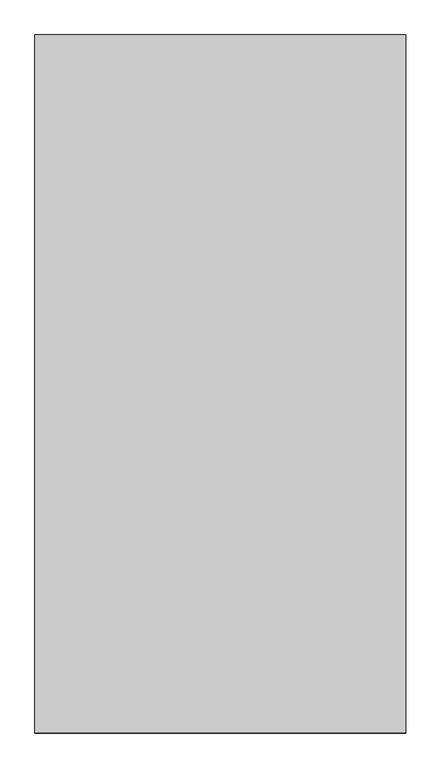
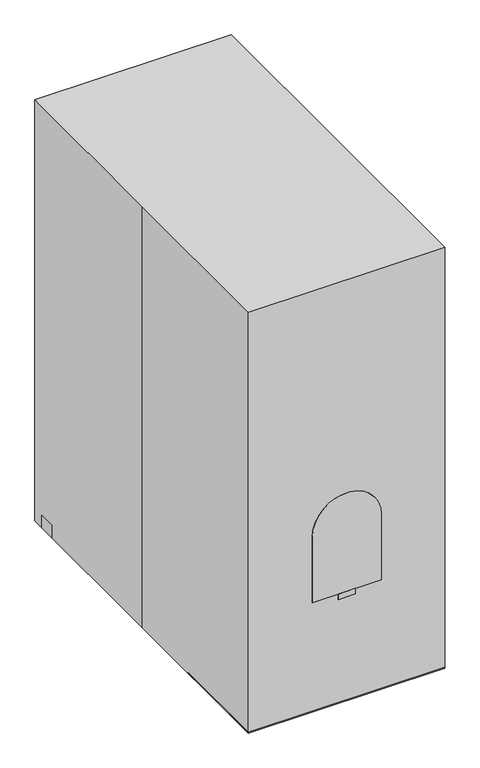
"""IFC4 building model written with IfcOpenShell, lengths in millimetres: proxy geometry, M8133 - Ergometer, Upper Body : M8133 - Ergometer, Upper Body."""

from ifc_helpers import new_model, si_unit, point, frame, frame_2d, origin, origin_with_axes, place, context, project, spatial, polyline, circle_curve, trimmed, segment, composite_curve, outline, extrude, faceted_brep, source, transform, mapped, element, save
from ifc_brep_helpers import plane_surface, cylinder_surface, revolved_surface, advanced_brep


def specialty_equipment_9e477837(model_context):
    return source(origin(), model_context, "Body", "SolidModel", [
        faceted_brep([(-152.4, -762.0, 457.2), (152.4, -762.0, 457.2), (152.4, -762.0, 508.0), (38.1, -762.0, 508.0), (38.1, -762.0, 482.6226424), (-38.1, -762.0, 482.6226424), (-38.1, -762.0, 508.0), (-152.4, -762.0, 508.0), (-152.4, -457.2, 457.2), (-152.4, -457.2, 508.0), (152.4, -457.2, 508.0), (152.4, -457.2, 457.2), (-38.1, -812.8, 508.0), (38.1, -812.8, 508.0), (-38.1, -812.8, 482.6226424), (38.1, -812.8, 482.6226424)], [[[0, 1, 2, 3, 4, 5, 6, 7]], [[8, 9, 10, 11]], [[1, 0, 8, 11]], [[2, 1, 11, 10]], [[10, 9, 7, 6, 12, 13, 3, 2]], [[0, 7, 9, 8]], [[14, 5, 4, 15]], [[13, 12, 14, 15]], [[3, 13, 15, 4]], [[12, 6, 5, 14]]]),
        advanced_brep(
        [(-76.2, 42.1480335, 1174.2765056), (-76.2, 59.4642449, 1191.592717), (-76.2, 212.6832937, 1038.3736683), (-76.2, 195.3670823, 1021.0574568), (-76.2, 46.8398769, 1180.5508736), (-76.2, 59.5398769, 1180.5508736), (-76.2, 207.9914503, 1032.0993003), (-76.2, 195.2914503, 1032.0993003), (-63.5, 42.1480335, 1174.2765056), (-63.5, 195.3670823, 1021.0574568), (-63.5, 212.6832937, 1038.3736683), (-63.5, 59.4642449, 1191.592717), (-63.5, 46.8398769, 1180.5508736), (-63.5, 59.5398769, 1180.5508736), (-165.1, 207.9914503, 1032.0993003), (-165.1, 195.2914503, 1032.0993003)],
        [
            (0, 1, circle_curve(frame((-76.2, 53.1898769, 1180.5508736), z_axis=(-1.0, 0.0, 0.0), x_axis=(0.0, 1.0, 0.0)), 12.7)),
            (1, 2),
            (2, 3, circle_curve(frame((-76.2, 201.6414503, 1032.0993003), z_axis=(-1.0, 0.0, 0.0), x_axis=(0.0, 1.0, 0.0)), 12.7)),
            (3, 0),
            (4, 5, circle_curve(frame((-76.2, 53.1898769, 1180.5508736), z_axis=(1.0, 0.0, 0.0), x_axis=(0.0, 1.0, 0.0)), 6.35)),
            (5, 4, circle_curve(frame((-76.2, 53.1898769, 1180.5508736), z_axis=(1.0, 0.0, 0.0), x_axis=(0.0, 1.0, 0.0)), 6.35)),
            (6, 7, circle_curve(frame((-76.2, 201.6414503, 1032.0993003), z_axis=(1.0, 0.0, 0.0), x_axis=(0.0, 1.0, 0.0)), 6.35)),
            (7, 6, circle_curve(frame((-76.2, 201.6414503, 1032.0993003), z_axis=(1.0, 0.0, 0.0), x_axis=(0.0, 1.0, 0.0)), 6.35)),
            (8, 9),
            (9, 10, circle_curve(frame((-63.5, 201.6414503, 1032.0993003), z_axis=(1.0, 0.0, 0.0), x_axis=(0.0, 1.0, 0.0)), 12.7)),
            (10, 11),
            (11, 8, circle_curve(frame((-63.5, 53.1898769, 1180.5508736), z_axis=(1.0, 0.0, 0.0), x_axis=(0.0, 1.0, 0.0)), 12.7)),
            (12, 13, circle_curve(frame((-63.5, 53.1898769, 1180.5508736), z_axis=(-1.0, 0.0, 0.0), x_axis=(0.0, 1.0, 0.0)), 6.35)),
            (13, 12, circle_curve(frame((-63.5, 53.1898769, 1180.5508736), z_axis=(-1.0, 0.0, 0.0), x_axis=(0.0, 1.0, 0.0)), 6.35)),
            (3, 9),
            (8, 0),
            (2, 10),
            (1, 11),
            (5, 13),
            (12, 4),
            (14, 15, circle_curve(frame((-165.1, 201.6414503, 1032.0993003), z_axis=(-1.0, 0.0, 0.0), x_axis=(0.0, 1.0, 0.0)), 6.35)),
            (15, 14, circle_curve(frame((-165.1, 201.6414503, 1032.0993003), z_axis=(-1.0, 0.0, 0.0), x_axis=(0.0, 1.0, 0.0)), 6.35)),
            (15, 7),
            (6, 14),
        ],
        [
            plane_surface(frame((-76.2, 65.8898769, 1180.5508736), z_axis=(-1.0, 0.0, 0.0), x_axis=(0.0, 0.0, -1.0))),
            plane_surface(frame((-63.5, 65.8898769, 1180.5508736), z_axis=(1.0, 0.0, 0.0), x_axis=(0.0, 0.0, 1.0))),
            plane_surface(frame((-76.2, 195.3670823, 1021.0574568), z_axis=(0.0, -0.7071067811865492, -0.7071067811865458), x_axis=(1.0, 0.0, 0.0))),
            cylinder_surface(frame((-63.5, 201.6414503, 1032.0993003), z_axis=(-1.0, 0.0, 0.0), x_axis=(0.0, 1.0, 0.0)), 12.7),
            plane_surface(frame((-76.2, 59.4642449, 1191.592717), z_axis=(0.0, 0.7071067811865492, 0.7071067811865458), x_axis=(1.0, 0.0, 0.0))),
            cylinder_surface(frame((-63.5, 53.1898769, 1180.5508736), z_axis=(-1.0, 0.0, 0.0), x_axis=(0.0, 1.0, 0.0)), 12.7),
            revolved_surface(polyline([(-63.5, 59.5398769, 1180.5508736), (-76.2, 59.5398769, 1180.5508736)]), (0.0, 53.1898769, 1180.5508736), (1.0, 0.0, 0.0)),
            plane_surface(frame((-165.1, 207.9914503, 1032.0993003), z_axis=(-1.0, 0.0, 0.0), x_axis=(0.0, 0.0, -1.0))),
            cylinder_surface(frame((-63.5, 201.6414503, 1032.0993003), z_axis=(-1.0, 0.0, 0.0), x_axis=(0.0, 1.0, 0.0)), 6.35),
        ],
        [
            (0, [[1, 2, 3, 4], [5, 6], [7, 8]]),
            (1, [[9, 10, 11, 12], [13, 14]]),
            (2, [[-4, 15, -9, 16]]),
            (3, [[-3, 17, -10, -15]]),
            (4, [[-2, 18, -11, -17]]),
            (5, [[-1, -16, -12, -18]]),
            (6, [[-6, 19, -13, 20]]),
            (6, [[-5, -20, -14, -19]]),
            (7, [[21, 22]]),
            (8, [[-22, 23, -7, 24]]),
            (8, [[-21, -24, -8, -23]]),
        ],
    ),
        advanced_brep(
        [(165.1, 207.9914503, 1032.0993003), (165.1, 195.2914503, 1032.0993003), (63.5, 42.1480335, 1174.2765056), (63.5, 59.4642449, 1191.592717), (63.5, 212.6832937, 1038.3736683), (63.5, 195.3670823, 1021.0574568), (63.5, 46.8398769, 1180.5508736), (63.5, 59.5398769, 1180.5508736), (76.2, 207.9914503, 1032.0993003), (76.2, 195.2914503, 1032.0993003), (76.2, 42.1480335, 1174.2765056), (76.2, 195.3670823, 1021.0574568), (76.2, 212.6832937, 1038.3736683), (76.2, 59.4642449, 1191.592717), (76.2, 46.8398769, 1180.5508736), (76.2, 59.5398769, 1180.5508736)],
        [
            (0, 1, circle_curve(frame((165.1, 201.6414503, 1032.0993003), z_axis=(1.0, 0.0, 0.0), x_axis=(0.0, 1.0, 0.0)), 6.35)),
            (1, 0, circle_curve(frame((165.1, 201.6414503, 1032.0993003), z_axis=(1.0, 0.0, 0.0), x_axis=(0.0, 1.0, 0.0)), 6.35)),
            (2, 3, circle_curve(frame((63.5, 53.1898769, 1180.5508736), z_axis=(-1.0, 0.0, 0.0), x_axis=(0.0, 1.0, 0.0)), 12.7)),
            (3, 4),
            (4, 5, circle_curve(frame((63.5, 201.6414503, 1032.0993003), z_axis=(-1.0, 0.0, 0.0), x_axis=(0.0, 1.0, 0.0)), 12.7)),
            (5, 2),
            (6, 7, circle_curve(frame((63.5, 53.1898769, 1180.5508736), z_axis=(1.0, 0.0, 0.0), x_axis=(0.0, 1.0, 0.0)), 6.35)),
            (7, 6, circle_curve(frame((63.5, 53.1898769, 1180.5508736), z_axis=(1.0, 0.0, 0.0), x_axis=(0.0, 1.0, 0.0)), 6.35)),
            (0, 8),
            (8, 9, circle_curve(frame((76.2, 201.6414503, 1032.0993003), z_axis=(1.0, 0.0, 0.0), x_axis=(0.0, 1.0, 0.0)), 6.35)),
            (9, 1),
            (9, 8, circle_curve(frame((76.2, 201.6414503, 1032.0993003), z_axis=(1.0, 0.0, 0.0), x_axis=(0.0, 1.0, 0.0)), 6.35)),
            (10, 11),
            (11, 12, circle_curve(frame((76.2, 201.6414503, 1032.0993003), z_axis=(1.0, 0.0, 0.0), x_axis=(0.0, 1.0, 0.0)), 12.7)),
            (12, 13),
            (13, 10, circle_curve(frame((76.2, 53.1898769, 1180.5508736), z_axis=(1.0, 0.0, 0.0), x_axis=(0.0, 1.0, 0.0)), 12.7)),
            (14, 15, circle_curve(frame((76.2, 53.1898769, 1180.5508736), z_axis=(-1.0, 0.0, 0.0), x_axis=(0.0, 1.0, 0.0)), 6.35)),
            (15, 14, circle_curve(frame((76.2, 53.1898769, 1180.5508736), z_axis=(-1.0, 0.0, 0.0), x_axis=(0.0, 1.0, 0.0)), 6.35)),
            (10, 2),
            (5, 11),
            (4, 12),
            (3, 13),
            (14, 6),
            (7, 15),
        ],
        [
            plane_surface(frame((165.1, 207.9914503, 1032.0993003), z_axis=(1.0, 0.0, 0.0), x_axis=(0.0, 0.0, 1.0))),
            plane_surface(frame((63.5, 207.9914503, 1032.0993003), z_axis=(-1.0, 0.0, 0.0), x_axis=(0.0, 0.0, -1.0))),
            cylinder_surface(frame((63.5, 201.6414503, 1032.0993003), z_axis=(1.0, 0.0, 0.0), x_axis=(0.0, 1.0, 0.0)), 6.35),
            plane_surface(frame((76.2, 51.6829843, 1164.7415548), z_axis=(1.0, 0.0, 0.0), x_axis=(0.0, 0.7071067811865458, -0.7071067811865492))),
            plane_surface(frame((76.2, 42.1480335, 1174.2765056), z_axis=(0.0, -0.7071067811865492, -0.7071067811865458), x_axis=(-1.0, 0.0, 0.0))),
            cylinder_surface(frame((63.5, 201.6414503, 1032.0993003), z_axis=(1.0, 0.0, 0.0), x_axis=(0.0, 1.0, 0.0)), 12.7),
            plane_surface(frame((76.2, 212.6832937, 1038.3736683), z_axis=(0.0, 0.7071067811865492, 0.7071067811865458), x_axis=(-1.0, 0.0, 0.0))),
            cylinder_surface(frame((63.5, 53.1898769, 1180.5508736), z_axis=(1.0, 0.0, 0.0), x_axis=(0.0, 1.0, 0.0)), 12.7),
            revolved_surface(polyline([(63.5, 59.5398769, 1180.5508736), (76.2, 59.5398769, 1180.5508736)]), (0.0, 53.1898769, 1180.5508736), (-1.0, 0.0, 0.0)),
        ],
        [
            (0, [[1, 2]]),
            (1, [[3, 4, 5, 6], [7, 8]]),
            (2, [[-1, 9, 10, 11]]),
            (2, [[-2, -11, 12, -9]]),
            (3, [[13, 14, 15, 16], [-10, -12], [17, 18]]),
            (4, [[-13, 19, -6, 20]]),
            (5, [[-14, -20, -5, 21]]),
            (6, [[-15, -21, -4, 22]]),
            (7, [[-16, -22, -3, -19]]),
            (8, [[-17, 23, -8, 24]]),
            (8, [[-18, -24, -7, -23]]),
        ],
    ),
        advanced_brep(
        [(50.8, 0.0, 1270.0), (50.8, 0.0, 1066.8), (50.8, 475.1958334, 1117.6), (50.8, 406.4, 1270.0), (50.8, 487.68, 1432.56), (50.8, 468.63, 1426.21), (50.8, 196.9503327, 1426.21), (50.8, 171.5503327, 1400.81), (50.8, 171.5503327, 1327.1834442), (50.8, 59.5398769, 1180.5508736), (50.8, 46.8398769, 1180.5508736), (-50.8, 475.1958334, 1117.6), (-50.8, 0.0, 1066.8), (-50.8, 0.0, 1270.0), (-50.8, 171.5503327, 1327.1834442), (-50.8, 171.5503327, 1400.81), (-50.8, 196.9503327, 1426.21), (-50.8, 468.63, 1426.21), (-50.8, 487.68, 1432.56), (-50.8, 406.4, 1270.0), (-50.8, 46.8398769, 1180.5508736), (-50.8, 59.5398769, 1180.5508736), (76.2, 406.4, 1270.0), (76.2, 812.8, 1270.0), (-76.2, 406.4, 1270.0), (-76.2, 812.8, 1270.0), (63.5, 486.8027128, 1108.1016793), (63.5, 541.769184, 1078.455696), (-63.5, 541.769184, 1078.455696), (-63.5, 486.8027128, 1108.1016793), (63.5, 634.9505562, 53.975), (63.5, 685.7505562, 53.975), (-63.5, 685.7505562, 53.975), (-63.5, 634.9505562, 53.975), (76.2, 46.8398769, 1180.5508736), (76.2, 59.5398769, 1180.5508736), (-76.2, 46.8398769, 1180.5508736), (-76.2, 59.5398769, 1180.5508736)],
        [
            (0, 1, circle_curve(frame((50.8, 33.8666667, 1168.4), z_axis=(1.0, 0.0, 0.0), x_axis=(0.0, 1.0, 0.0)), 107.0958034)),
            (1, 2),
            (2, 3, circle_curve(frame((50.8, 609.6, 1270.0), z_axis=(-1.0, 0.0, 0.0), x_axis=(0.0, 1.0, 0.0)), 203.2)),
            (3, 4, circle_curve(frame((50.8, 609.6, 1270.0), z_axis=(-1.0, 0.0, 0.0), x_axis=(0.0, 1.0, 0.0)), 203.2)),
            (4, 5),
            (5, 6),
            (6, 7, circle_curve(frame((50.8, 196.9503327, 1400.81), z_axis=(1.0, 0.0, 0.0), x_axis=(0.0, 1.0, 0.0)), 25.4)),
            (7, 8),
            (8, 0),
            (9, 10, circle_curve(frame((50.8, 53.1898769, 1180.5508736), z_axis=(-1.0, 0.0, 0.0), x_axis=(0.0, 1.0, 0.0)), 6.35)),
            (10, 9, circle_curve(frame((50.8, 53.1898769, 1180.5508736), z_axis=(-1.0, 0.0, 0.0), x_axis=(0.0, 1.0, 0.0)), 6.35)),
            (11, 12),
            (12, 13, circle_curve(frame((-50.8, 33.8666667, 1168.4), z_axis=(-1.0, 0.0, 0.0), x_axis=(0.0, 1.0, 0.0)), 107.0958034)),
            (13, 14),
            (14, 15),
            (15, 16, circle_curve(frame((-50.8, 196.9503327, 1400.81), z_axis=(-1.0, 0.0, 0.0), x_axis=(0.0, 1.0, 0.0)), 25.4)),
            (16, 17),
            (17, 18),
            (18, 19, circle_curve(frame((-50.8, 609.6, 1270.0), z_axis=(1.0, 0.0, 0.0), x_axis=(0.0, 1.0, 0.0)), 203.2)),
            (19, 11, circle_curve(frame((-50.8, 609.6, 1270.0), z_axis=(1.0, 0.0, 0.0), x_axis=(0.0, 1.0, 0.0)), 203.2)),
            (20, 21, circle_curve(frame((-50.8, 53.1898769, 1180.5508736), z_axis=(1.0, 0.0, 0.0), x_axis=(0.0, 1.0, 0.0)), 6.35)),
            (21, 20, circle_curve(frame((-50.8, 53.1898769, 1180.5508736), z_axis=(1.0, 0.0, 0.0), x_axis=(0.0, 1.0, 0.0)), 6.35)),
            (13, 0),
            (8, 14),
            (4, 18),
            (17, 5),
            (12, 1),
            (11, 2),
            (22, 23, circle_curve(frame((76.2, 609.6, 1270.0), z_axis=(1.0, 0.0, 0.0), x_axis=(0.0, 1.0, 0.0)), 203.2)),
            (23, 22, circle_curve(frame((76.2, 609.6, 1270.0), z_axis=(1.0, 0.0, 0.0), x_axis=(0.0, 1.0, 0.0)), 203.2)),
            (24, 25, circle_curve(frame((-76.2, 609.6, 1270.0), z_axis=(-1.0, 0.0, 0.0), x_axis=(0.0, 1.0, 0.0)), 203.2)),
            (25, 24, circle_curve(frame((-76.2, 609.6, 1270.0), z_axis=(-1.0, 0.0, 0.0), x_axis=(0.0, 1.0, 0.0)), 203.2)),
            (22, 3),
            (19, 24),
            (25, 23),
            (26, 27, circle_curve(frame((63.5, 609.6, 1270.0), z_axis=(1.0, 0.0, 0.0), x_axis=(0.0, 1.0, 0.0)), 203.2)),
            (27, 28),
            (28, 29, circle_curve(frame((-63.5, 609.6, 1270.0), z_axis=(-1.0, 0.0, 0.0), x_axis=(0.0, 1.0, 0.0)), 203.2)),
            (29, 26),
            (7, 15),
            (16, 6),
            (30, 31),
            (31, 27),
            (26, 30),
            (32, 33),
            (33, 29),
            (28, 32),
            (33, 30),
            (32, 31),
            (34, 35, circle_curve(frame((76.2, 53.1898769, 1180.5508736), z_axis=(1.0, 0.0, 0.0), x_axis=(0.0, 1.0, 0.0)), 6.35)),
            (35, 34, circle_curve(frame((76.2, 53.1898769, 1180.5508736), z_axis=(1.0, 0.0, 0.0), x_axis=(0.0, 1.0, 0.0)), 6.35)),
            (34, 10),
            (9, 35),
            (36, 37, circle_curve(frame((-76.2, 53.1898769, 1180.5508736), z_axis=(-1.0, 0.0, 0.0), x_axis=(0.0, 1.0, 0.0)), 6.35)),
            (37, 36, circle_curve(frame((-76.2, 53.1898769, 1180.5508736), z_axis=(-1.0, 0.0, 0.0), x_axis=(0.0, 1.0, 0.0)), 6.35)),
            (37, 21),
            (20, 36),
        ],
        [
            plane_surface(frame((50.8, 812.8, 1270.0), z_axis=(1.0, 0.0, 0.0), x_axis=(0.0, 0.0, -1.0))),
            plane_surface(frame((-50.8, 812.8, 1270.0), z_axis=(-1.0, 0.0, 0.0), x_axis=(0.0, 0.0, 1.0))),
            plane_surface(frame((50.8, 487.68, 1432.56), z_axis=(0.0, -0.3162277660168353, 0.9486832980505148), x_axis=(-1.0, 0.0, 0.0))),
            cylinder_surface(frame((-50.8, 33.8666667, 1168.4), z_axis=(1.0, 0.0, 0.0), x_axis=(0.0, 1.0, 0.0)), 107.0958034),
            plane_surface(frame((50.8, 0.0, 1066.8), z_axis=(0.0, 0.10629761849075979, -0.9943343584042507), x_axis=(-1.0, 0.0, 0.0))),
            plane_surface(frame((76.2, 812.8, 1270.0), z_axis=(1.0, 0.0, 0.0), x_axis=(0.0, 0.0, 1.0))),
            plane_surface(frame((-76.2, 812.8, 1270.0), z_axis=(-1.0, 0.0, 0.0), x_axis=(0.0, 0.0, -1.0))),
            cylinder_surface(frame((-76.2, 609.6, 1270.0), z_axis=(1.0, 0.0, 0.0), x_axis=(0.0, 1.0, 0.0)), 203.2),
            plane_surface(frame((50.8, 171.5503327, 1400.81), z_axis=(0.0, -1.0, 0.0), x_axis=(-1.0, 0.0, 0.0))),
            plane_surface(frame((50.8, 468.63, 1426.21), z_axis=(0.0, 0.0, 1.0), x_axis=(-1.0, 0.0, 0.0))),
            cylinder_surface(frame((-50.8, 196.9503327, 1400.81), z_axis=(1.0, 0.0, 0.0), x_axis=(0.0, 1.0, 0.0)), 25.4),
            plane_surface(frame((63.5, 536.2678109, 1117.6), z_axis=(1.0, 0.0, 0.0), x_axis=(0.0, -1.0, 0.0))),
            plane_surface(frame((-63.5, 536.2678109, 1117.6), z_axis=(-1.0, 0.0, 0.0), x_axis=(0.0, 1.0, 0.0))),
            plane_surface(frame((63.5, 485.4678109, 1117.6), z_axis=(0.0, -0.9902680687415706, -0.1391731009600634), x_axis=(-1.0, 0.0, 0.0))),
            plane_surface(frame((63.5, 634.9505562, 53.975), z_axis=(0.0, 0.0, -1.0), x_axis=(-1.0, 0.0, 0.0))),
            plane_surface(frame((63.5, 685.7505562, 53.975), z_axis=(0.0, 0.9902680687415706, 0.13917310096006333), x_axis=(-1.0, 0.0, 0.0))),
            plane_surface(frame((76.2, 59.5398769, 1180.5508736), z_axis=(1.0, 0.0, 0.0), x_axis=(0.0, 0.0, 1.0))),
            cylinder_surface(frame((50.8, 53.1898769, 1180.5508736), z_axis=(1.0, 0.0, 0.0), x_axis=(0.0, 1.0, 0.0)), 6.35),
            plane_surface(frame((-76.2, 59.5398769, 1180.5508736), z_axis=(-1.0, 0.0, 0.0), x_axis=(0.0, 0.0, -1.0))),
            cylinder_surface(frame((-50.8, 53.1898769, 1180.5508736), z_axis=(-1.0, 0.0, 0.0), x_axis=(0.0, 1.0, 0.0)), 6.35),
        ],
        [
            (0, [[1, 2, 3, 4, 5, 6, 7, 8, 9], [10, 11]]),
            (1, [[12, 13, 14, 15, 16, 17, 18, 19, 20], [21, 22]]),
            (2, [[23, -9, 24, -14]]),
            (2, [[25, -18, 26, -5]]),
            (3, [[-1, -23, -13, 27]]),
            (4, [[-2, -27, -12, 28]]),
            (5, [[29, 30]]),
            (6, [[31, 32]]),
            (7, [[-29, 33, -3, -28, -20, 34, -32, 35], [36, 37, 38, 39]]),
            (7, [[-30, -35, -31, -34, -19, -25, -4, -33]]),
            (8, [[-8, 40, -15, -24]]),
            (9, [[-6, -26, -17, 41]]),
            (10, [[-7, -41, -16, -40]]),
            (11, [[42, 43, -36, 44]]),
            (12, [[45, 46, -38, 47]]),
            (13, [[48, -44, -39, -46]]),
            (14, [[-42, -48, -45, 49]]),
            (15, [[-49, -47, -37, -43]]),
            (16, [[50, 51]]),
            (17, [[-50, 52, -10, 53]]),
            (17, [[-51, -53, -11, -52]]),
            (18, [[54, 55]]),
            (19, [[-55, 56, -21, 57]]),
            (19, [[-54, -57, -22, -56]]),
        ],
    ),
        extrude(outline(polyline([(431.8, 762.0), (431.8, 685.7505562), (-431.8, 685.7505562), (-431.8, 762.0), (431.8, 762.0)])), origin_with_axes(), (0.0, 0.0, 1.0), 57.15),
        extrude(outline(composite_curve([segment(polyline([(812.8, -152.4), (508.0, -152.4), (508.0, 152.4), (812.8, 152.4)]), True, "CONTINUOUS"), segment(trimmed(circle_curve(frame_2d((812.8, 0.0)), 152.4), [point((812.8, 152.4))], [point((812.8, -152.4))], False, "CARTESIAN"), True, "CONTINUOUS")], self_intersect=False)), frame((0.0, -812.8, 0.0), z_axis=(0.0, 1.0, 0.0), x_axis=(0.0, 0.0, 1.0)), (0.0, 0.0, 1.0), 50.8),
        extrude(outline(polyline([(-555.0633542, 60.325), (-612.775, 60.325), (-668.5521438, 457.2), (-610.840498, 457.2), (-555.0633542, 60.325)])), frame((-38.1, 0.0, 0.0), z_axis=(1.0, 0.0, 0.0), x_axis=(0.0, 1.0, 0.0)), (0.0, 0.0, 1.0), 76.2),
        extrude(outline(polyline([(3.175, -69.85), (3.175, -63.5), (53.975, -63.5), (53.975, 63.5), (3.175, 63.5), (3.175, 69.85), (60.325, 69.85), (60.325, -69.85), (3.175, -69.85)])), frame((0.0, -660.4, 0.0), z_axis=(0.0, 1.0, 0.0), x_axis=(0.0, 0.0, 1.0)), (0.0, 0.0, 1.0), 152.4),
        extrude(outline(polyline([(431.8, -812.8), (-431.8, -812.8), (-431.8, -355.6), (431.8, -355.6), (431.8, -812.8)])), origin_with_axes(), (0.0, 0.0, 1.0), 3.175),
        extrude(outline(polyline([(63.5, 685.7505562), (63.5, -584.2), (-63.5, -584.2), (-63.5, 685.7505562), (63.5, 685.7505562)])), frame((0.0, 0.0, 3.175), z_axis=(0.0, 0.0, 1.0), x_axis=(1.0, 0.0, 0.0)), (0.0, 0.0, 1.0), 50.8),
        extrude(outline(polyline([(-431.8, 812.8), (431.8, 812.8), (431.8, -812.8), (-431.8, -812.8), (-431.8, 0.0), (-431.8, 812.8)])), origin_with_axes(), (0.0, 0.0, 1.0), 1955.8),
    ])


if __name__ == "__main__":
    model = new_model("IFC4")
    model_context = context("Model", 3, world=origin())
    ifc_project = project(units=[si_unit("LENGTHUNIT", "METRE", prefix="MILLI")], contexts=[model_context])
    site = spatial("IfcSite", under=ifc_project)
    building = spatial("IfcBuilding", under=site)
    placement = place(None, origin())
    specialty_equipment_shape = specialty_equipment_9e477837(model_context)
    element("IfcBuildingElementProxy", 1, Name="M8133 - Ergometer, Upper Body : M8133 - Ergometer, Upper Body", ObjectType="M8133 - Ergometer, Upper Body : M8133 - Ergometer, Upper Body", at=placement, inside=building, context=model_context, shape_type="MappedRepresentation", body=[
        mapped(specialty_equipment_shape, transform((0.0, 0.0, 0.0), x_axis=(1.0, 0.0, 0.0), y_axis=(0.0, 1.0, 0.0), z_axis=(0.0, 0.0, 1.0))),
    ])
    save(model, "model.ifc")

# Revit data of these elements
# Type "M8133 - Ergometer, Upper Body : M8133 - Ergometer, Upper Body"
#   Watts2 = "0"
#   Watts1 = "360"
#   Unit_Issue = "EA"
#   UTIL_6_Misc = "-"
#   UTIL_5_NonMedGas = "-"
#   UTIL_4_MiscGas = "-"
#   UTIL_3_MedGas = "-"
#   UTIL_2_Elec = "A"
#   UTIL_1_WaterDrain = "-"
#   Nomenclature = "Ergometer, Upper Body"
#   NSN = "6530"
#   Location [instance default] = ""
#   JSN = "M8133"
#   Fund_Source_VA = "-"
#   Fund_Source_Navy = "-"
#   Fund_Source_Army = "-"
#   Fund_Source_AF = "-"
#   ELEC_Volts2 = "0"
#   ELEC_Volts1 = "120"
#   ELEC_Phase2 = "0"
#   ELEC_Phase1 = "1"
#   ELEC_HertzSwitch = "0"
#   ELEC_HertzDependent = "-1"
#   ELEC_Hertz = "60"
#   ELEC_Amps2 = "0"
#   ELEC_Amps1 = "3"
#   DetailDescription = "Ergometer for measuring upper body exertion during an exercise regimen. The unit consists of a seat and a hand crank mechanism at shoulder height. The unit is used for physical rehabilitation protocols and stress testing. The unit quantifiably measures the effort exerted by the patient."
#   CAT_VA = "C"
#   CAT_Navy = "C"
#   CAT_IHS = "-"
#   CAT_Army = "C"
#   CAT_AF = "C"
#   BTUperhour = "0"
#   Weight_IP = 250
#   DIM_Width_IP = 2' - 10"
#   DIM_Height_IP = 6' - 5"
#   DIM_Depth_IP = 5' - 4"
# Element 1 (IfcBuildingElementProxy, "M8133 - Ergometer, Upper Body : M8133 - Ergometer, Upper Body")
#   Location = "OPTM1"
#   Materials on its faces: "EquipSpace"
# Materials
#   "EquipSpace": class "Unassigned", colour RGB 221 217 195, transparency 0.5
